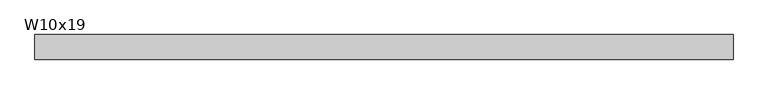
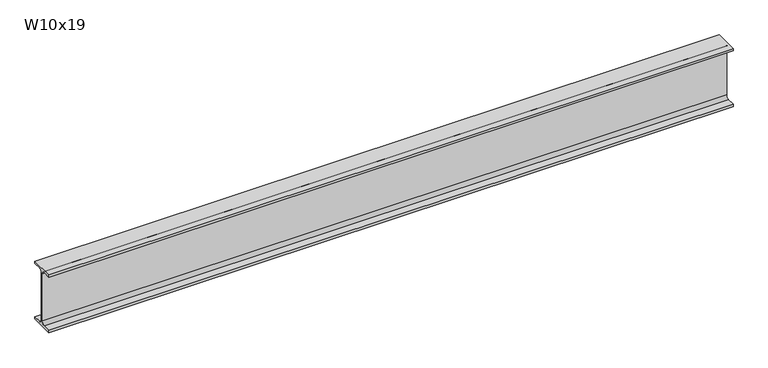
"""IFC4 building model written with IfcOpenShell, lengths in millimetres: beam geometry, RME W-Wide Flange : W10x19."""

from ifc_helpers import new_model, si_unit, point, frame, frame_2d, origin, place, context, project, spatial, polyline, circle_curve, trimmed, segment, composite_curve, outline, extrude, source, transform, mapped, element, save


def w10x19_dd4a4555(model_context):
    return source(origin(), model_context, "Body", "SweptSolid", [
        extrude(outline(composite_curve([segment(polyline([(51.054, -119.507), (51.054, -129.54), (-51.054, -129.54), (-51.054, -119.507), (-16.9545, -119.507)]), True, "CONTINUOUS"), segment(trimmed(circle_curve(frame_2d((-16.9545, -105.7275)), 13.7795), [point((-16.9545, -119.507))], [point((-3.175, -105.7275))], True, "CARTESIAN"), True, "CONTINUOUS"), segment(polyline([(-3.175, -105.7275), (-3.175, 105.7275)]), True, "CONTINUOUS"), segment(trimmed(circle_curve(frame_2d((-16.9545, 105.7275)), 13.7795), [point((-3.175, 105.7275))], [point((-16.9545, 119.507))], True, "CARTESIAN"), True, "CONTINUOUS"), segment(polyline([(-16.9545, 119.507), (-51.054, 119.507), (-51.054, 129.54), (51.054, 129.54), (51.054, 119.507), (16.9545, 119.507)]), True, "CONTINUOUS"), segment(trimmed(circle_curve(frame_2d((16.9545, 105.7275)), 13.7795), [point((16.9545, 119.507))], [point((3.175, 105.7275))], True, "CARTESIAN"), True, "CONTINUOUS"), segment(polyline([(3.175, 105.7275), (3.175, -105.7275)]), True, "CONTINUOUS"), segment(trimmed(circle_curve(frame_2d((16.9545, -105.7275)), 13.7795), [point((3.175, -105.7275))], [point((16.9545, -119.507))], True, "CARTESIAN"), True, "CONTINUOUS"), segment(polyline([(16.9545, -119.507), (51.054, -119.507)]), True, "CONTINUOUS")], self_intersect=False)), frame((-1450.3277687, 0.0, 0.0), z_axis=(1.0, 0.0, 0.0), x_axis=(0.0, 1.0, 0.0)), (0.0, 0.0, 1.0), 2898.8567108),
    ])


if __name__ == "__main__":
    model = new_model("IFC4")
    model_context = context("Model", 3, world=origin())
    ifc_project = project(units=[si_unit("LENGTHUNIT", "METRE", prefix="MILLI")], contexts=[model_context])
    site = spatial("IfcSite", under=ifc_project)
    building = spatial("IfcBuilding", under=site)
    placement = place(None, origin())
    w10x19_shape = w10x19_dd4a4555(model_context)
    element("IfcBeam", 1, ObjectType="RME W-Wide Flange : W10x19", at=placement, inside=building, context=model_context, shape_type="MappedRepresentation", body=[
        mapped(w10x19_shape, transform((0.0, 0.0, 0.0), x_axis=(1.0, 0.0, 0.0), y_axis=(0.0, 1.0, 0.0), z_axis=(0.0, 0.0, 1.0))),
    ])
    save(model, "model.ifc")

# Revit data of these elements
# Type "RME W-Wide Flange : W10x19"
#   WELD P [instance default] = ""
#   WELD LE [instance default] = ""
#   WELD D [instance default] = ""
#   TOP SECTION SIZE [instance default] = ""
#   TOP SECTION LENGTH [instance default] = ""
#   REMARKS [instance default] = ""
#   REINF TYPE [instance default] = ""
#   Nominal Size = "W24"
#   End Bearing Capacity [instance default] = ""
#   BOT SECTION SIZE [instance default] = ""
#   BOT SECTION LENGTH [instance default] = ""
#   Assembly Code = "B10"
#   W = 19
#   Start Extension Calculation [instance default] = 10' - 0"
#   Start Extension [instance default] = -0' - 0 1/2"
#   End Extension Calculation [instance default] = 10' - 0"
#   End Extension [instance default] = -0' - 0 1/2"
#   Length [instance default] = 5' - 0"
#   bf = 0' - 4.02"
#   d = 0' - 10.2"
#   k = 0' - 0 15/16"
#   k2 = 0' - 0.5425"
#   tf = 0' - 0.395"
#   tw = 0' - 0 1/4"
#   A = 0.0390278 SF
#   Structural Material [instance default] = Metal - Steel - ASTM A992
# Element 1 (IfcBeam, "RME W-Wide Flange : W10x19")
#   Length = 9' - 7.72607"
#   Materials on its faces: "Metal - Steel - ASTM A992"
# Materials
#   "Metal - Steel - ASTM A992": class "Metal", colour RGB 255 128 0, transparency 0
